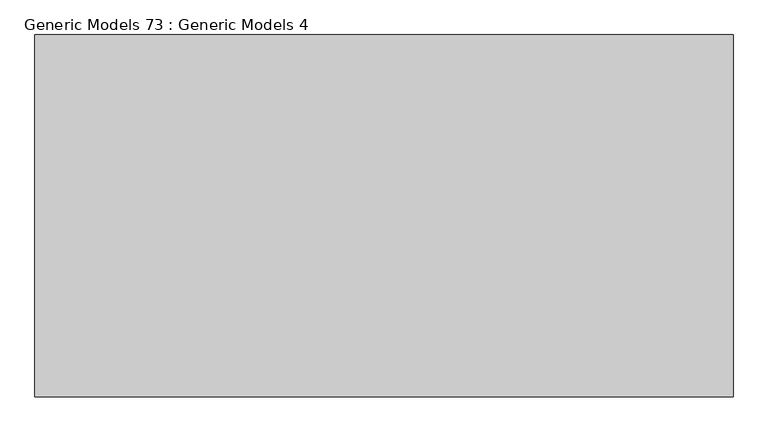
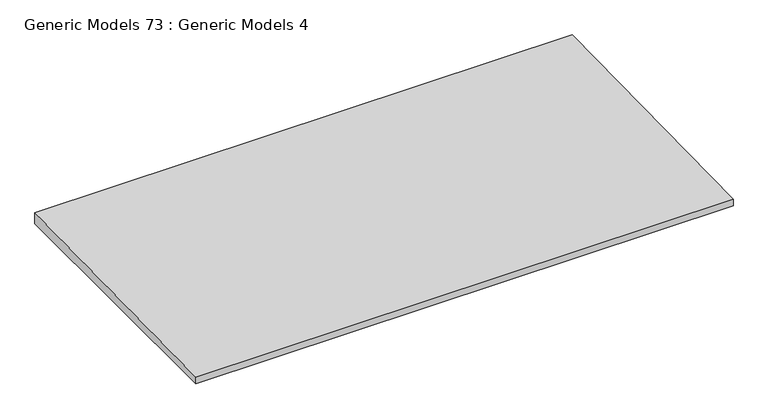
"""IFC4 building model written with IfcOpenShell, lengths in millimetres: proxy geometry, Generic Models 73 : Generic Models 4."""

from ifc_helpers import new_model, si_unit, frame, origin, place, context, project, spatial, polyline, outline, extrude, source, transform, mapped, element, save


def generic_models_73_generic_models_4_64a28f80(model_context):
    return source(origin(), model_context, "Body", "SweptSolid", [
        extrude(outline(polyline([(-11722.3554199, 123145.296), (-11722.3554199, 123235.0484874), (-8057.0818256, 123299.0260759), (-8057.0818256, 123145.296), (-11722.3554199, 123145.296)])), frame((23168.0573109, 0.0, 0.0), z_axis=(1.0, 0.0, 0.0), x_axis=(0.0, 1.0, 0.0)), (0.0, 0.0, 1.0), 7061.0177484),
    ])


if __name__ == "__main__":
    model = new_model("IFC4")
    model_context = context("Model", 3, world=origin())
    ifc_project = project(units=[si_unit("LENGTHUNIT", "METRE", prefix="MILLI")], contexts=[model_context])
    site = spatial("IfcSite", under=ifc_project)
    building = spatial("IfcBuilding", under=site)
    placement = place(None, origin())
    generic_models_73_generic_models_4_shape = generic_models_73_generic_models_4_64a28f80(model_context)
    element("IfcBuildingElementProxy", 1, Name="Generic Models 73 : Generic Models 4", ObjectType="Generic Models 73 : Generic Models 4", at=placement, inside=building, context=model_context, shape_type="MappedRepresentation", body=[
        mapped(generic_models_73_generic_models_4_shape, transform((0.0, 0.0, 0.0), x_axis=(1.0, 0.0, 0.0), y_axis=(0.0, 1.0, 0.0), z_axis=(0.0, 0.0, 1.0))),
    ])
    save(model, "model.ifc")

# Revit data of these elements
# Element 1 (IfcBuildingElementProxy, "Generic Models 73 : Generic Models 4")
#   Materials on its faces: "_CONCRETE SLAB W/ WIRE MESH (SEE STRUCT. DWGS) - SLOPE 1% AWAY FROM BUILDING"
# Materials
#   "_CONCRETE SLAB W/ WIRE MESH (SEE STRUCT. DWGS) - SLOPE 1% AWAY FROM BUILDING": class "Generic", colour RGB 191 191 191, transparency 0, Cost = 0
